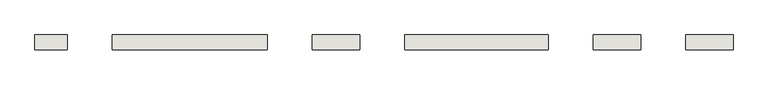
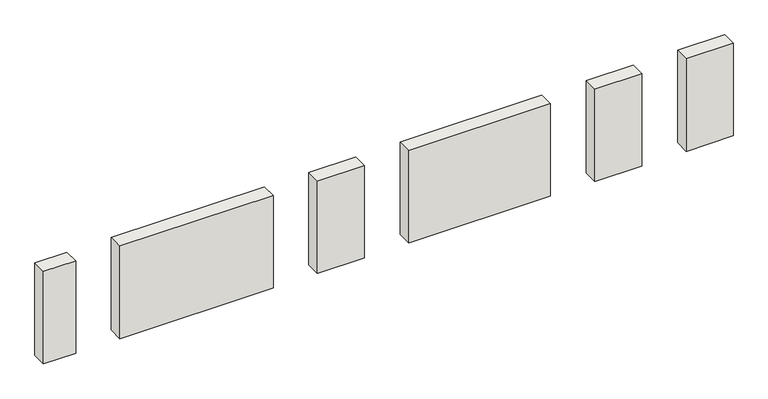
"""IFC4 building model written with IfcOpenShell, lengths in millimetres: wall geometry, 0_3d."""

import ifcopenshell
import ifcopenshell.guid

model = None  # the IFC model being written
_history = None  # IfcOwnerHistory: only IFC2X3 demands one
_inside = {}  # id of a spatial element -> (the spatial element, [elements in it])
_under = {}  # id of a project, library or spatial element -> (it, [spatial elements below it])
_declared = {}  # id of a project -> (the project, [libraries it declares])
_typed = {}  # id of a type object -> (the type object, [elements of that type])
_made_of = {}  # id of a material, layer set ... -> (it, [elements and type objects made of it])


def new_model(schema):
    """Start an empty IFC model of exactly this schema.

    Asked for "IFC4X3", IfcOpenShell would pick the latest addendum, in which some entities
    have other attributes; the version numbers below select the first issue.
    IFC2X3 requires an IfcOwnerHistory on every rooted entity: one is made here for all.
    """
    global model, _history
    if schema == "IFC4X3":
        model = ifcopenshell.file(schema_version=(4, 3, 0, 0))
    else:
        model = ifcopenshell.file(schema=schema)
    _inside.clear()
    _under.clear()
    _declared.clear()
    _typed.clear()
    _made_of.clear()
    _history = None
    if model.schema == "IFC2X3":
        org = make("IfcOrganization", Name="unknown")
        user = make(
            "IfcPersonAndOrganization",
            ThePerson=make("IfcPerson", FamilyName="unknown"),
            TheOrganization=org,
        )
        app = make(
            "IfcApplication",
            ApplicationDeveloper=org,
            Version="unknown",
            ApplicationFullName="unknown",
            ApplicationIdentifier="unknown",
        )
        _history = make(
            "IfcOwnerHistory",
            OwningUser=user,
            OwningApplication=app,
            ChangeAction="ADDED",
            CreationDate=0,
        )
    return model


def make(cls, **values):
    """One entity of the class cls with the attributes given. An attribute that is None is left unset."""
    return model.create_entity(
        cls, **{name: value for name, value in values.items() if value is not None}
    )


def rooted(cls, **values):
    """An entity with a GlobalId (a new one), such as an element, a storey or a relation."""
    return make(cls, GlobalId=ifcopenshell.guid.new(), OwnerHistory=_history, **values)


def si_unit(unit_type, name, prefix=None):
    """IfcSIUnit, for example si_unit("LENGTHUNIT", "METRE", prefix="MILLI")."""
    return make("IfcSIUnit", UnitType=unit_type, Prefix=prefix, Name=name)


def assignment(units):
    """IfcUnitAssignment: the units of a project."""
    return None if units is None else make("IfcUnitAssignment", Units=units)


def point(xyz):
    """IfcCartesianPoint."""
    return None if xyz is None else make("IfcCartesianPoint", Coordinates=xyz)


def direction(xyz):
    """IfcDirection."""
    return None if xyz is None else make("IfcDirection", DirectionRatios=xyz)


def frame(location, z_axis=None, x_axis=None):
    """IfcAxis2Placement3D, a coordinate frame: its origin and axes. An axis left out is left unset."""
    return make(
        "IfcAxis2Placement3D",
        Location=point(location),
        Axis=direction(z_axis),
        RefDirection=direction(x_axis),
    )


def origin():
    """The frame at (0, 0, 0) with its axes left unset."""
    return frame((0.0, 0.0, 0.0))


def origin_with_axes():
    """The frame at (0, 0, 0) with the z axis (0, 0, 1) and the x axis (1, 0, 0) written out."""
    return frame((0.0, 0.0, 0.0), z_axis=(0.0, 0.0, 1.0), x_axis=(1.0, 0.0, 0.0))


def place(relative_to, where):
    """IfcLocalPlacement: puts the frame where relative to a parent placement (None: the world)."""
    return make(
        "IfcLocalPlacement", PlacementRelTo=relative_to, RelativePlacement=where
    )


def context(
    kind, dimensions, precision=None, world=None, true_north=None, identifier=None
):
    """IfcGeometricRepresentationContext, for example the 3D "Model" context."""
    return make(
        "IfcGeometricRepresentationContext",
        ContextIdentifier=identifier,
        ContextType=kind,
        CoordinateSpaceDimension=dimensions,
        Precision=precision,
        WorldCoordinateSystem=world,
        TrueNorth=true_north,
    )


def project(units=None, contexts=None):
    """IfcProject with its units and contexts."""
    return rooted(
        "IfcProject",
        Name="project",
        RepresentationContexts=contexts,
        UnitsInContext=assignment(units),
    )


def spatial(cls, under=None, at=None, **own):
    """A site, building, storey or space (cls), placed at a placement, below another one or the project."""
    s = rooted(cls, ObjectPlacement=at, **own)
    if under is not None:
        _under.setdefault(under.id(), (under, []))[1].append(s)
    return s


def polyline(points):
    """IfcPolyline through the points."""
    return make("IfcPolyline", Points=[point(p) for p in points])


def outline(outer, holes=None, kind="AREA"):
    """IfcArbitraryClosedProfileDef: a profile drawn as a closed curve; with holes, ...WithVoids."""
    if holes is None:
        return make("IfcArbitraryClosedProfileDef", ProfileType=kind, OuterCurve=outer)
    return make(
        "IfcArbitraryProfileDefWithVoids",
        ProfileType=kind,
        OuterCurve=outer,
        InnerCurves=holes,
    )


def extrude(swept, where, along, depth):
    """IfcExtrudedAreaSolid: the profile swept, set in the frame where, extruded along a direction by depth."""
    return make(
        "IfcExtrudedAreaSolid",
        SweptArea=swept,
        Position=where,
        ExtrudedDirection=direction(along),
        Depth=depth,
    )


def shape(context_of_items, identifier, shape_type, items):
    """IfcShapeRepresentation: the items that make up one representation, for example the "Body"."""
    return make(
        "IfcShapeRepresentation",
        ContextOfItems=context_of_items,
        RepresentationIdentifier=identifier,
        RepresentationType=shape_type,
        Items=items,
    )


def source(mapping_origin, context_of_items, identifier, shape_type, items):
    """IfcRepresentationMap: a shape defined once, which mapped items show again and again."""
    return make(
        "IfcRepresentationMap",
        MappingOrigin=mapping_origin,
        MappedRepresentation=shape(context_of_items, identifier, shape_type, items),
    )


def transform(
    local_origin,
    x_axis=None,
    y_axis=None,
    z_axis=None,
    scale=None,
    scale2=None,
    scale3=None,
    uniform=True,
):
    """IfcCartesianTransformationOperator3D, or its non-uniform kind. x_axis, y_axis, z_axis: its Axis1, 2, 3."""
    if uniform:
        return make(
            "IfcCartesianTransformationOperator3D",
            Axis1=direction(x_axis),
            Axis2=direction(y_axis),
            LocalOrigin=point(local_origin),
            Scale=scale,
            Axis3=direction(z_axis),
        )
    return make(
        "IfcCartesianTransformationOperator3DnonUniform",
        Axis1=direction(x_axis),
        Axis2=direction(y_axis),
        LocalOrigin=point(local_origin),
        Scale=scale,
        Axis3=direction(z_axis),
        Scale2=scale2,
        Scale3=scale3,
    )


def mapped(mapping_source, mapping_target):
    """IfcMappedItem: shows the shape of a source again, moved by a transform."""
    return make(
        "IfcMappedItem", MappingSource=mapping_source, MappingTarget=mapping_target
    )


def made_of(thing, what):
    """Note that an element or type object is made of a material, layer set ...; save() writes the relation."""
    if what is not None:
        _made_of.setdefault(what.id(), (what, []))[1].append(thing)
    return thing


def element(
    cls,
    number,
    at=None,
    inside=None,
    cuts=None,
    type_object=None,
    material=None,
    context=None,
    identifier="Body",
    shape_type=None,
    held_by="IfcProductDefinitionShape",
    body=None,
    shapes=None,
    **own,
):
    """One element of the class cls, such as IfcWall. Its Tag is "e" and its number.

    at: its placement. inside: the storey or other place that contains it. cuts: it is an
    opening in that element (IfcRelVoidsElement). A single representation is given by context,
    identifier, shape_type and body (its items); several are given by shapes. held_by: the class
    of the entity that holds the representations. save() writes the other relations.
    """
    e = rooted(cls, Tag="e%d" % number, ObjectPlacement=at, **own)
    if body is not None:
        shapes = [shape(context, identifier, shape_type, body)]
    if shapes is not None:
        e.Representation = make(held_by, Representations=shapes)
    if inside is not None:
        _inside.setdefault(inside.id(), (inside, []))[1].append(e)
    if cuts is not None:
        rooted(
            "IfcRelVoidsElement", RelatingBuildingElement=cuts, RelatedOpeningElement=e
        )
    if type_object is not None:
        _typed.setdefault(type_object.id(), (type_object, []))[1].append(e)
    return made_of(e, material)


def aggregate(whole, parts):
    """IfcRelAggregates: a whole, such as a stair, and the parts it consists of."""
    return rooted("IfcRelAggregates", RelatingObject=whole, RelatedObjects=parts)


def save(model, path):
    """Write the relations noted so far, then the file.

    IfcRelAggregates (storeys below a building ...), IfcRelContainedInSpatialStructure (elements
    in a storey), IfcRelDefinesByType, IfcRelAssociatesMaterial and IfcRelDeclares: one each for
    every whole, place, type object, material and project.
    """
    for whole, parts in _under.values():
        aggregate(whole, parts)
    for where, things in _inside.values():
        rooted(
            "IfcRelContainedInSpatialStructure",
            RelatedElements=things,
            RelatingStructure=where,
        )
    for kind, things in _typed.values():
        rooted("IfcRelDefinesByType", RelatedObjects=things, RelatingType=kind)
    for what, things in _made_of.values():
        rooted("IfcRelAssociatesMaterial", RelatedObjects=things, RelatingMaterial=what)
    for by, libraries in _declared.values():
        rooted("IfcRelDeclares", RelatingContext=by, RelatedDefinitions=libraries)
    model.write(path)


def wall_6d111875(model_context):
    return source(origin(), model_context, "Body", "SweptSolid", [
        extrude(outline(polyline([(819.602585, 380.0), (819.602585, 0.0), (0.0, 0.0), (0.0, 380.0), (819.602585, 380.0)])), origin_with_axes(), (0.0, 0.0, 1.0), 2500.0),
        extrude(outline(polyline([(5865.3619019, 380.0), (5865.3619019, 0.0), (1954.602585, 0.0), (1954.602585, 380.0), (5865.3619019, 380.0)])), origin_with_axes(), (0.0, 0.0, 1.0), 2500.0),
        extrude(outline(polyline([(7000.3619019, 0.0), (7000.3619019, 380.0), (8199.9644869, 380.0), (8199.9644869, 0.0), (7000.3619019, 0.0)])), origin_with_axes(), (0.0, 0.0, 1.0), 2500.0),
        extrude(outline(polyline([(9334.9644869, 0.0), (9334.9644869, 380.0), (12954.7954033, 380.0), (12954.7954033, 0.0), (9334.9644869, 0.0)])), origin_with_axes(), (0.0, 0.0, 1.0), 2500.0),
        extrude(outline(polyline([(15287.8619019, 380.0), (15287.8619019, 0.0), (14089.7954033, 0.0), (14089.7954033, 380.0), (15287.8619019, 380.0)])), origin_with_axes(), (0.0, 0.0, 1.0), 2500.0),
        extrude(outline(polyline([(16422.8619019, 0.0), (16422.8619019, 380.0), (17622.8619019, 380.0), (17622.8619019, 0.0), (16422.8619019, 0.0)])), origin_with_axes(), (0.0, 0.0, 1.0), 2500.0),
    ])


if __name__ == "__main__":
    model = new_model("IFC4")
    model_context = context("Model", 3, world=origin())
    ifc_project = project(units=[si_unit("LENGTHUNIT", "METRE", prefix="MILLI")], contexts=[model_context])
    site = spatial("IfcSite", under=ifc_project)
    building = spatial("IfcBuilding", under=site)
    placement = place(None, origin())
    wall_shape = wall_6d111875(model_context)
    element("IfcWall", 1, ObjectType="0_3d", at=placement, inside=building, context=model_context, shape_type="MappedRepresentation", body=[
        mapped(wall_shape, transform((0.0, 0.0, 0.0), x_axis=(1.0, 0.0, 0.0), y_axis=(0.0, 1.0, 0.0), z_axis=(0.0, 0.0, 1.0))),
    ])
    save(model, "model.ifc")

# Revit data of these elements
# Element 1 (IfcWall, "0_3d")
#   Materials on its faces: "holzschalung"
# Materials
#   "holzschalung": class "Unassigned", colour RGB 128 128 128, transparency 0
